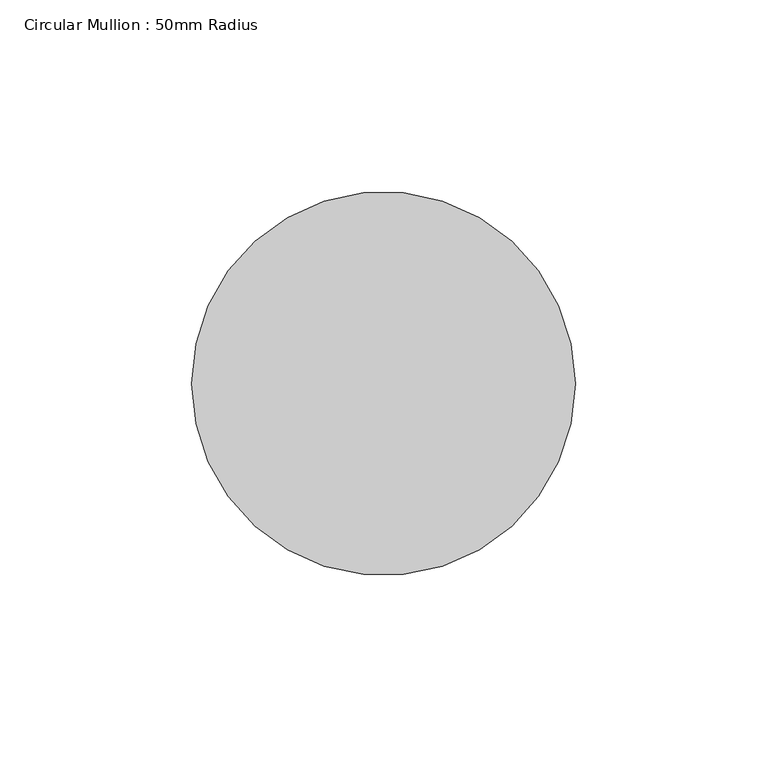
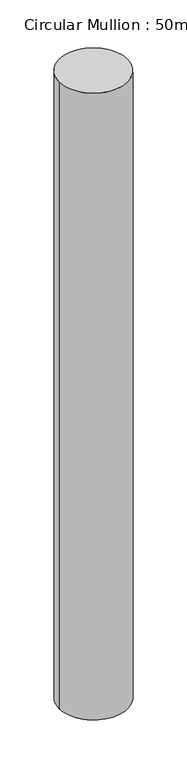
"""IFC4 building model written with IfcOpenShell, lengths in millimetres: member geometry, Circular Mullion : 50mm Radius."""

from ifc_helpers import new_model, si_unit, point, frame, origin, origin_2d, place, context, project, spatial, circle_curve, trimmed, segment, composite_curve, outline, extrude, source, transform, mapped, element, save


def circular_mullion_50mm_radius_93a68f6d(model_context):
    return source(origin(), model_context, "Body", "SweptSolid", [
        extrude(outline(composite_curve([segment(trimmed(circle_curve(origin_2d(), 50.0), [point((50.0, 0.0))], [point((-50.0, 0.0))], False, "CARTESIAN"), True, "CONTINUOUS"), segment(trimmed(circle_curve(origin_2d(), 50.0), [point((-50.0, 0.0))], [point((50.0, 0.0))], False, "CARTESIAN"), True, "CONTINUOUS")], self_intersect=False)), frame((0.0, 0.0, -966.7685218), z_axis=(0.0, 0.0, 1.0), x_axis=(1.0, 0.0, 0.0)), (0.0, 0.0, 1.0), 966.7685218),
    ])


if __name__ == "__main__":
    model = new_model("IFC4")
    model_context = context("Model", 3, world=origin())
    ifc_project = project(units=[si_unit("LENGTHUNIT", "METRE", prefix="MILLI")], contexts=[model_context])
    site = spatial("IfcSite", under=ifc_project)
    building = spatial("IfcBuilding", under=site)
    placement = place(None, origin())
    circular_mullion_50mm_radius_shape = circular_mullion_50mm_radius_93a68f6d(model_context)
    element("IfcMember", 1, ObjectType="Circular Mullion : 50mm Radius", at=placement, inside=building, context=model_context, shape_type="MappedRepresentation", body=[
        mapped(circular_mullion_50mm_radius_shape, transform((0.0, 0.0, 0.0), x_axis=(1.0, 0.0, 0.0), y_axis=(0.0, 1.0, 0.0), z_axis=(0.0, 0.0, 1.0))),
    ])
    save(model, "model.ifc")

# Revit data of these elements
# Type "Circular Mullion : 50mm Radius"
#   built-in parameter 1007350 = 0.164042 (stored number, unit not read)
# Element 1 (IfcMember, "Circular Mullion : 50mm Radius")
#   Materials on its faces: "Aluminium"
# Materials
#   "Aluminium": class "Metal", colour RGB 247 247 247, transparency 0, Description = "Aluminium 6061", Cost = 0
